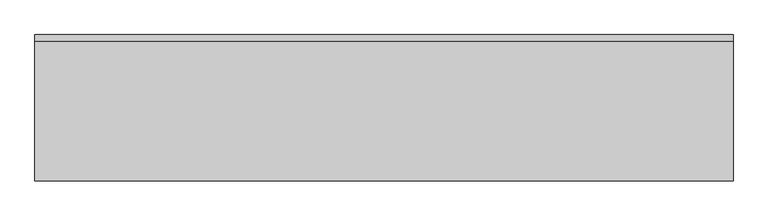
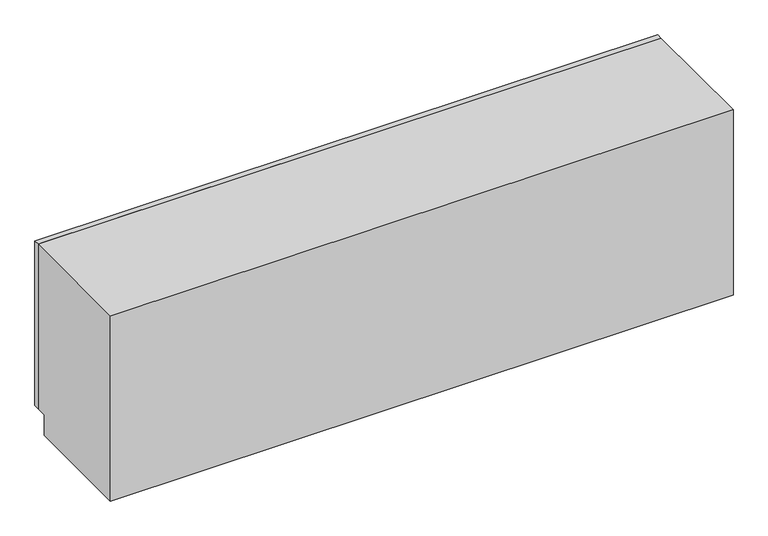
"""IFC4 building model written with IfcOpenShell, lengths in millimetres: furniture geometry, OD_CW_Base Cabinet : OD_CW_Base Cabinet."""

from ifc_helpers import new_model, si_unit, frame, origin, place, context, project, spatial, polyline, outline, extrude, source, transform, mapped, element, save


def furniture_fafa2a9b(model_context):
    return source(origin(), model_context, "Body", "SweptSolid", [
        extrude(outline(polyline([(18.7377049, -25.4), (18.7377049, 0.0), (2923.5832917, 0.0), (2923.5832917, -25.4), (18.7377049, -25.4)])), frame((0.0, 0.0, 101.6), z_axis=(0.0, 0.0, 1.0), x_axis=(1.0, 0.0, 0.0)), (0.0, 0.0, 1.0), 812.8),
        extrude(outline(polyline([(-25.4, 914.4), (-25.4, 101.6), (-76.2, 101.6), (-76.2, 0.0), (-609.6, 0.0), (-609.6, 914.4), (-25.4, 914.4)])), frame((18.7377049, 0.0, 0.0), z_axis=(1.0, 0.0, 0.0), x_axis=(0.0, 1.0, 0.0)), (0.0, 0.0, 1.0), 2904.8455868),
    ])


if __name__ == "__main__":
    model = new_model("IFC4")
    model_context = context("Model", 3, world=origin())
    ifc_project = project(units=[si_unit("LENGTHUNIT", "METRE", prefix="MILLI")], contexts=[model_context])
    site = spatial("IfcSite", under=ifc_project)
    building = spatial("IfcBuilding", under=site)
    placement = place(None, origin())
    furniture_shape = furniture_fafa2a9b(model_context)
    element("IfcFurniture", 1, ObjectType="OD_CW_Base Cabinet : OD_CW_Base Cabinet", at=placement, inside=building, context=model_context, shape_type="MappedRepresentation", body=[
        mapped(furniture_shape, transform((0.0, 0.0, 0.0), x_axis=(1.0, 0.0, 0.0), y_axis=(0.0, 1.0, 0.0), z_axis=(0.0, 0.0, 1.0))),
    ])
    save(model, "model.ifc")

# Revit data of these elements
# Type "OD_CW_Base Cabinet : OD_CW_Base Cabinet"
#   OD_CW_Width [instance default] = 2' - 10"
#   OD_CW_Length [instance default] = 8' - 0"
#   OD_CW_Height [instance default] = 2' - 3"
#   Depth = 2' - 0"
#   Height = 3' - 0"
#   Width = 4' - 0"
#   OD_CW_Material_Front Panel [instance default] = none
#   OD_CW_Material_Body [instance default] = none
# Element 1 (IfcFurniture, "OD_CW_Base Cabinet : OD_CW_Base Cabinet")
#   OD_CW_Width = 2' - 0"
#   OD_CW_Length = 9' - 6.364"
#   OD_CW_Height = 3' - 0"
#   OD_CW_Material_Body = PREP/MIXING AREA
#   Materials on its faces: "PREP/MIXING AREA", "CASEWORK"
# Materials
#   "PREP/MIXING AREA": class "Generic", colour RGB 181 181 181, transparency 0, Cost = 0
#   "CASEWORK": class "Generic", colour RGB 181 181 181, transparency 0, Cost = 0
